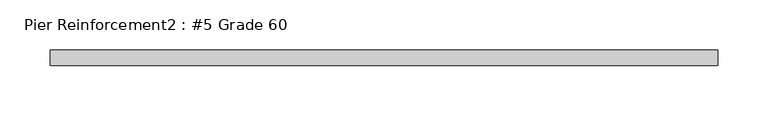
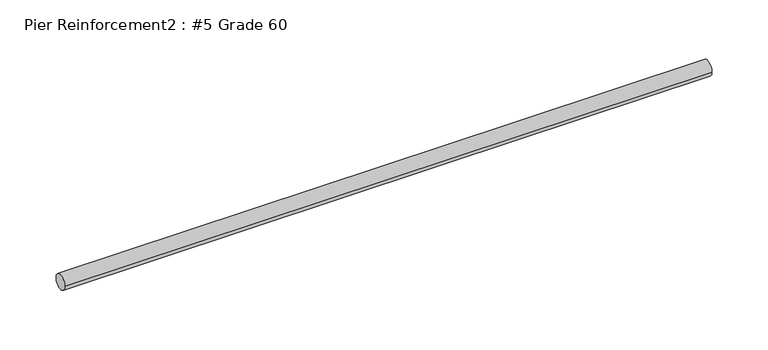
"""IFC4 building model written with IfcOpenShell, lengths in millimetres: proxy geometry, Pier Reinforcement2 : #5 Grade 60."""

from ifc_helpers import new_model, si_unit, point, frame, frame_2d, origin, place, context, project, spatial, circle_curve, trimmed, segment, composite_curve, outline, extrude, source, transform, mapped, element, save


def pier_reinforcement2_5_grade_60_756cefbf(model_context):
    return source(origin(), model_context, "Body", "SweptSolid", [
        extrude(outline(composite_curve([segment(trimmed(circle_curve(frame_2d((-531775.7413841, -55.5625)), 7.9375), [point((-531767.8038841, -55.5625))], [point((-531783.6788841, -55.5625))], False, "CARTESIAN"), True, "CONTINUOUS"), segment(trimmed(circle_curve(frame_2d((-531775.7413841, -55.5625)), 7.9375), [point((-531783.6788841, -55.5625))], [point((-531767.8038841, -55.5625))], False, "CARTESIAN"), True, "CONTINUOUS")], self_intersect=False)), frame((589567.2422365, 0.0, 0.0), z_axis=(1.0, 0.0, 0.0), x_axis=(0.0, 1.0, 0.0)), (0.0, 0.0, 1.0), 666.75),
    ])


if __name__ == "__main__":
    model = new_model("IFC4")
    model_context = context("Model", 3, world=origin())
    ifc_project = project(units=[si_unit("LENGTHUNIT", "METRE", prefix="MILLI")], contexts=[model_context])
    site = spatial("IfcSite", under=ifc_project)
    building = spatial("IfcBuilding", under=site)
    placement = place(None, origin())
    pier_reinforcement2_5_grade_60_shape = pier_reinforcement2_5_grade_60_756cefbf(model_context)
    element("IfcBuildingElementProxy", 1, Name="Pier Reinforcement2 : #5 Grade 60", ObjectType="Pier Reinforcement2 : #5 Grade 60", at=placement, inside=building, context=model_context, shape_type="MappedRepresentation", body=[
        mapped(pier_reinforcement2_5_grade_60_shape, transform((0.0, 0.0, 0.0), x_axis=(1.0, 0.0, 0.0), y_axis=(0.0, 1.0, 0.0), z_axis=(0.0, 0.0, 1.0))),
    ])
    save(model, "model.ifc")

# Revit data of these elements
# Element 1 (IfcBuildingElementProxy, "Pier Reinforcement2 : #5 Grade 60")
#   Materials on its faces: "#4 GR. 60 REINF. @ 16\" O.C. EW."
# Materials
#   "#4 GR. 60 REINF. @ 16\" O.C. EW.": class "Generic", colour RGB 84 83 81, transparency 0, Cost = 0
